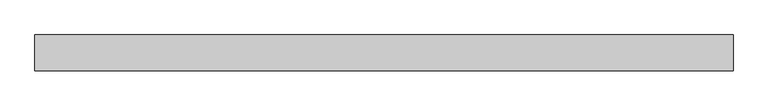
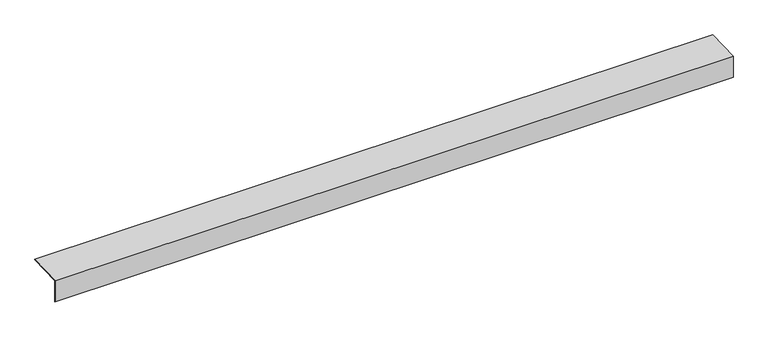
"""IFC4 building model written with IfcOpenShell, lengths in millimetres: proxy geometry, Generic Models 7:Generic Models 1:7:Generic Models 1:7 : Generic Models 7:Generic Models 1:337419:3 : Generic Models 7:Generic Models 1:7:Generic Models 1:7 : Generic Models 7:Generic Models 1:337419:315055."""

from ifc_helpers import new_model, si_unit, frame, origin, place, context, project, spatial, polyline, outline, extrude, source, transform, mapped, element, save


def generic_models_8323a79d(model_context):
    return source(origin(), model_context, "Body", "SweptSolid", [
        extrude(outline(polyline([(-579143.6477614, -81.7582633), (-579145.2352614, -81.7582633), (-579145.2352614, -1.1090262), (-579019.1128207, 4.1460755), (-579019.1128207, 2.5571981), (-579143.6477614, -2.6317578), (-579143.6477614, -81.7582633)])), frame((568001.5367239, 0.0, 0.0), z_axis=(1.0, 0.0, 0.0), x_axis=(0.0, 1.0, 0.0)), (0.0, 0.0, 1.0), 2451.1),
    ])


if __name__ == "__main__":
    model = new_model("IFC4")
    model_context = context("Model", 3, world=origin())
    ifc_project = project(units=[si_unit("LENGTHUNIT", "METRE", prefix="MILLI")], contexts=[model_context])
    site = spatial("IfcSite", under=ifc_project)
    building = spatial("IfcBuilding", under=site)
    placement = place(None, origin())
    generic_models_shape = generic_models_8323a79d(model_context)
    element("IfcBuildingElementProxy", 1, Name="Generic Models 7:Generic Models 1:7:Generic Models 1:7 : Generic Models 7:Generic Models 1:337419:3 : Generic Models 7:Generic Models 1:7:Generic Models 1:7 : Generic Models 7:Generic Models 1:337419:315055", ObjectType="Generic Models 7:Generic Models 1:7:Generic Models 1:7 : Generic Models 7:Generic Models 1:337419:3 : Generic Models 7:Generic Models 1:7:Generic Models 1:7 : Generic Models 7:Generic Models 1:337419:315055", at=placement, inside=building, context=model_context, shape_type="MappedRepresentation", body=[
        mapped(generic_models_shape, transform((0.0, 0.0, 0.0), x_axis=(1.0, 0.0, 0.0), y_axis=(0.0, 1.0, 0.0), z_axis=(0.0, 0.0, 1.0))),
    ])
    save(model, "model.ifc")

# Revit data of these elements
# Type "Generic Models 7:Generic Models 1:7:Generic Models 1:7 : Generic Models 7:Generic Models 1:337419:3 : Generic Models 7:Generic Models 1:7:Generic Models 1:7 : Generic Models 7:Generic Models 1:337419:315055"
#   NameOverride = "Generic Models 7:Generic Models 1:7:Generic Models 1:7 : Generic Models 7:Generic Models 1:337419:315055"
#   ObjectTypeOverride = "Generic Models 1:7 : Generic Models 7:Generic Models 1:337419"
#   Reference = "Generic Models 1"
#   Tag = "315055"
# Element 1 (IfcBuildingElementProxy, "Generic Models 7:Generic Models 1:7:Generic Models 1:7 : Generic Models 7:Generic Models 1:337419:3 : Generic Models 7:Generic Models 1:7:Generic Models 1:7 : Generic Models 7:Generic Models 1:337419:315055")
#   Materials on its faces: "16 GA. STAINLESS STEEL BRAKE METAL"
# Materials
#   "16 GA. STAINLESS STEEL BRAKE METAL": class "Unassigned", colour RGB 210 209 208, transparency 0, Cost = 0
